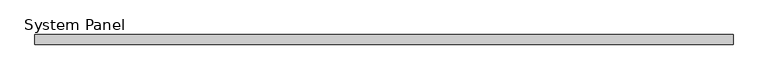
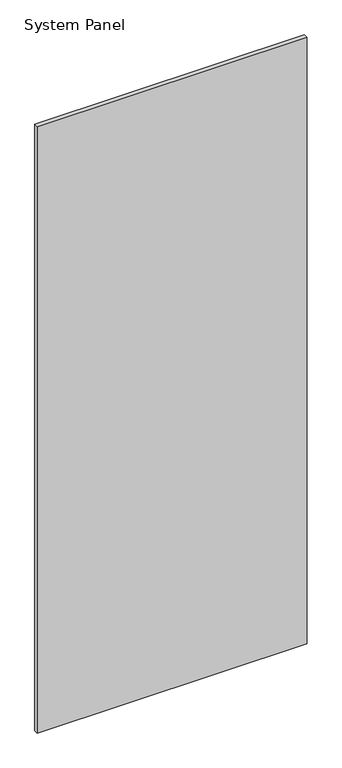
"""IFC4 building model written with IfcOpenShell, lengths in millimetres: plate geometry, System Panel : WWm-Glass-20mm-10mmOffset."""

from ifc_helpers import new_model, si_unit, origin, origin_with_axes, place, context, project, spatial, polyline, outline, extrude, source, transform, mapped, element, save


def system_panel_c2d77058(model_context):
    return source(origin(), model_context, "Body", "SweptSolid", [
        extrude(outline(polyline([(705.153103, 0.0), (-705.153103, 0.0), (-705.153103, 20.0), (705.153103, 20.0), (705.153103, 0.0)])), origin_with_axes(), (0.0, 0.0, 1.0), 3350.0),
    ])


if __name__ == "__main__":
    model = new_model("IFC4")
    model_context = context("Model", 3, world=origin())
    ifc_project = project(units=[si_unit("LENGTHUNIT", "METRE", prefix="MILLI")], contexts=[model_context])
    site = spatial("IfcSite", under=ifc_project)
    building = spatial("IfcBuilding", under=site)
    placement = place(None, origin())
    system_panel_shape = system_panel_c2d77058(model_context)
    element("IfcPlate", 1, ObjectType="System Panel : WWm-Glass-20mm-10mmOffset", at=placement, inside=building, context=model_context, shape_type="MappedRepresentation", body=[
        mapped(system_panel_shape, transform((0.0, 0.0, 0.0), x_axis=(1.0, 0.0, 0.0), y_axis=(0.0, 1.0, 0.0), z_axis=(0.0, 0.0, 1.0))),
    ])
    save(model, "model.ifc")

# Revit data of these elements
# Type "System Panel : WWm-Glass-20mm-10mmOffset"
#   Finish = ""
# Element 1 (IfcPlate, "System Panel : WWm-Glass-20mm-10mmOffset")
#   Materials on its faces: "WW-EC-GL-Storefront"
# Materials
#   "WW-EC-GL-Storefront": class "Glass", colour RGB 236 240 239, transparency 0.85, Description = "Storefront Glass", Cost = 0
